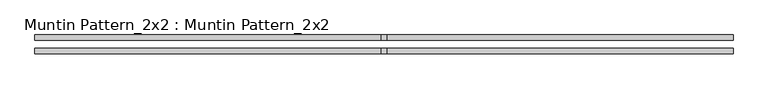
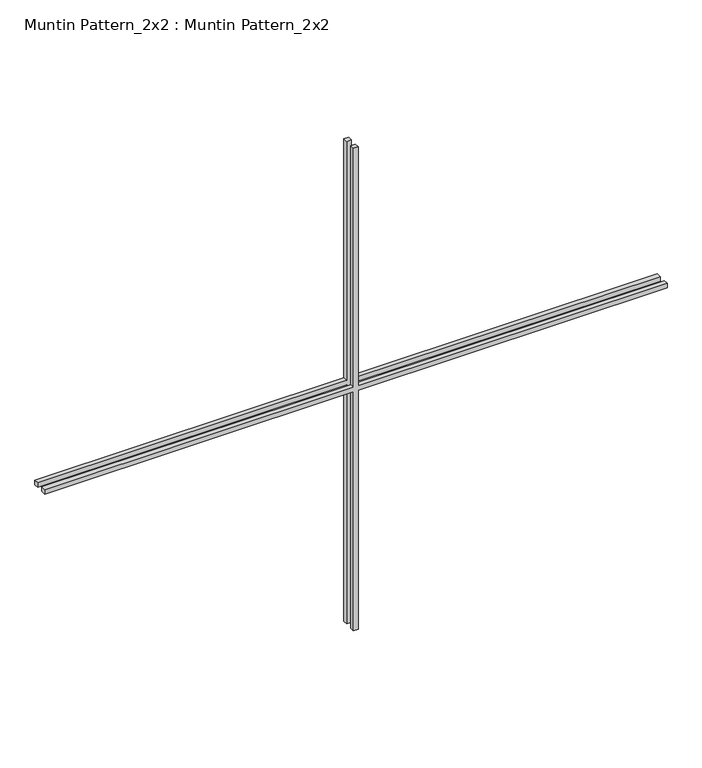
"""IFC4 building model written with IfcOpenShell, lengths in millimetres: proxy geometry, Muntin Pattern_2x2 : Muntin Pattern_2x2."""

from ifc_helpers import new_model, si_unit, frame, origin, place, context, project, spatial, polyline, outline, extrude, source, transform, mapped, element, save


def muntin_pattern_2x2_muntin_pattern_2x2_c30f9520(model_context):
    return source(origin(), model_context, "Body", "SweptSolid", [
        extrude(outline(polyline([(686.5, -6.35), (686.5, -830.15), (673.8, -830.15), (673.8, -6.35), (0.0, -6.35), (0.0, 6.35), (673.8, 6.35), (673.8, 830.15), (686.5, 830.15), (686.5, 6.35), (1360.3, 6.35), (1360.3, -6.35), (686.5, -6.35)])), frame((0.0, 9.525, 0.0), z_axis=(0.0, 1.0, 0.0), x_axis=(0.0, 0.0, 1.0)), (0.0, 0.0, 1.0), 12.7),
        extrude(outline(polyline([(686.5, -6.35), (686.5, -830.15), (673.8, -830.15), (673.8, -6.35), (0.0, -6.35), (0.0, 6.35), (673.8, 6.35), (673.8, 830.15), (686.5, 830.15), (686.5, 6.35), (1360.3, 6.35), (1360.3, -6.35), (686.5, -6.35)])), frame((0.0, -22.225, 0.0), z_axis=(0.0, 1.0, 0.0), x_axis=(0.0, 0.0, 1.0)), (0.0, 0.0, 1.0), 12.7),
    ])


if __name__ == "__main__":
    model = new_model("IFC4")
    model_context = context("Model", 3, world=origin())
    ifc_project = project(units=[si_unit("LENGTHUNIT", "METRE", prefix="MILLI")], contexts=[model_context])
    site = spatial("IfcSite", under=ifc_project)
    building = spatial("IfcBuilding", under=site)
    placement = place(None, origin())
    muntin_pattern_2x2_muntin_pattern_2x2_shape = muntin_pattern_2x2_muntin_pattern_2x2_c30f9520(model_context)
    element("IfcBuildingElementProxy", 1, Name="Muntin Pattern_2x2 : Muntin Pattern_2x2", ObjectType="Muntin Pattern_2x2 : Muntin Pattern_2x2", at=placement, inside=building, context=model_context, shape_type="MappedRepresentation", body=[
        mapped(muntin_pattern_2x2_muntin_pattern_2x2_shape, transform((0.0, 0.0, 0.0), x_axis=(1.0, 0.0, 0.0), y_axis=(0.0, 1.0, 0.0), z_axis=(0.0, 0.0, 1.0))),
    ])
    save(model, "model.ifc")

# Revit data of these elements
# Type "Muntin Pattern_2x2 : Muntin Pattern_2x2"
#   Width [instance default] = 121.92 cm
#   Thickness = 1.27 cm
#   Height [instance default] = 121.92 cm
#   Distance = 1.905 cm
#   Interior Material [instance default] = none
#   Exterior Material [instance default] = none
# Element 1 (IfcBuildingElementProxy, "Muntin Pattern_2x2 : Muntin Pattern_2x2")
#   Width = 166.03 cm
#   Height = 136.03 cm
#   Interior Material = Wood - Stained
#   Exterior Material = Clad - White
#   Materials on its faces: "Clad - White", "Wood - Stained"
# Materials
#   "Clad - White": class "Wood", colour RGB 242 242 238, transparency 0, Cost = 0
#   "Wood - Stained": class "Wood", colour RGB 224 178 126, transparency 0, Cost = 0
